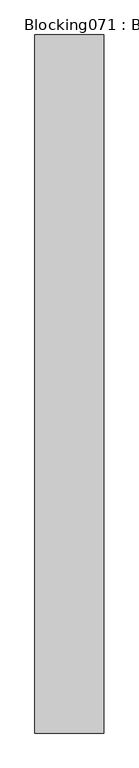
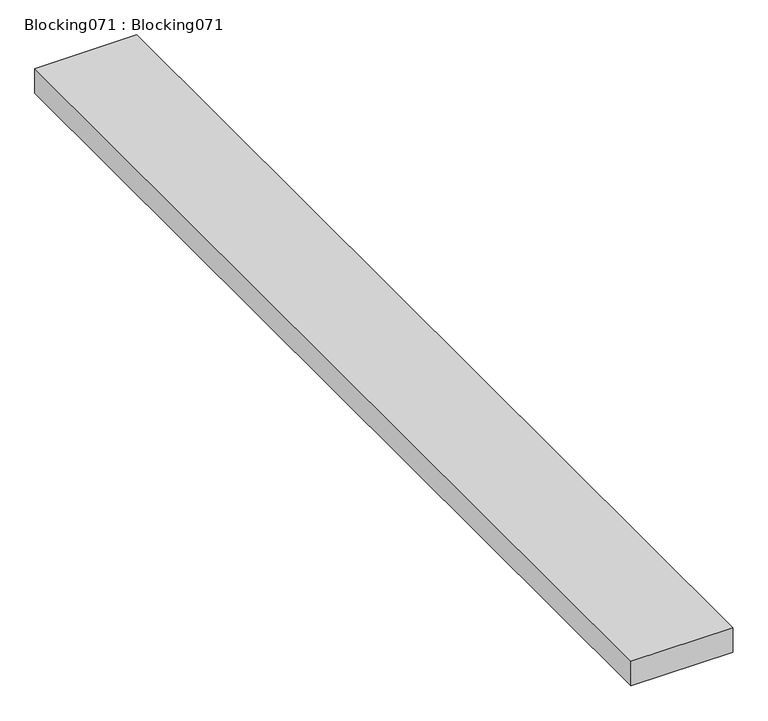
"""IFC4 building model written with IfcOpenShell, lengths in millimetres: proxy geometry, Blocking071 : Blocking071."""

from ifc_helpers import new_model, si_unit, frame, origin, place, context, project, spatial, polyline, outline, extrude, source, transform, mapped, element, save


def blocking071_blocking071_504c3a9e(model_context):
    return source(origin(), model_context, "Body", "SweptSolid", [
        extrude(outline(polyline([(-2567.3737014, -1052.8906574), (-2764.2237014, -1052.8906574), (-2764.2237014, 947.1093426), (-2567.3737014, 947.1093426), (-2567.3737014, -1052.8906574)])), frame((0.0, 0.0, 40131.746), z_axis=(0.0, 0.0, 1.0), x_axis=(1.0, 0.0, 0.0)), (0.0, 0.0, 1.0), 50.8),
    ])


if __name__ == "__main__":
    model = new_model("IFC4")
    model_context = context("Model", 3, world=origin())
    ifc_project = project(units=[si_unit("LENGTHUNIT", "METRE", prefix="MILLI")], contexts=[model_context])
    site = spatial("IfcSite", under=ifc_project)
    building = spatial("IfcBuilding", under=site)
    placement = place(None, origin())
    blocking071_blocking071_shape = blocking071_blocking071_504c3a9e(model_context)
    element("IfcBuildingElementProxy", 1, Name="Blocking071 : Blocking071", ObjectType="Blocking071 : Blocking071", at=placement, inside=building, context=model_context, shape_type="MappedRepresentation", body=[
        mapped(blocking071_blocking071_shape, transform((0.0, 0.0, 0.0), x_axis=(1.0, 0.0, 0.0), y_axis=(0.0, 1.0, 0.0), z_axis=(0.0, 0.0, 1.0))),
    ])
    save(model, "model.ifc")

# Revit data of these elements
# Type "Blocking071 : Blocking071"
#   NameOverride = "Blocking071"
# Element 1 (IfcBuildingElementProxy, "Blocking071 : Blocking071")
#   Materials on its faces: "WOOD BLOCKING AS REQUIRED"
# Materials
#   "WOOD BLOCKING AS REQUIRED": class "Unassigned", colour RGB 166 124 85, transparency 0, Cost = 0
